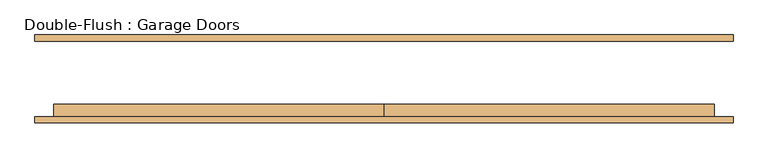
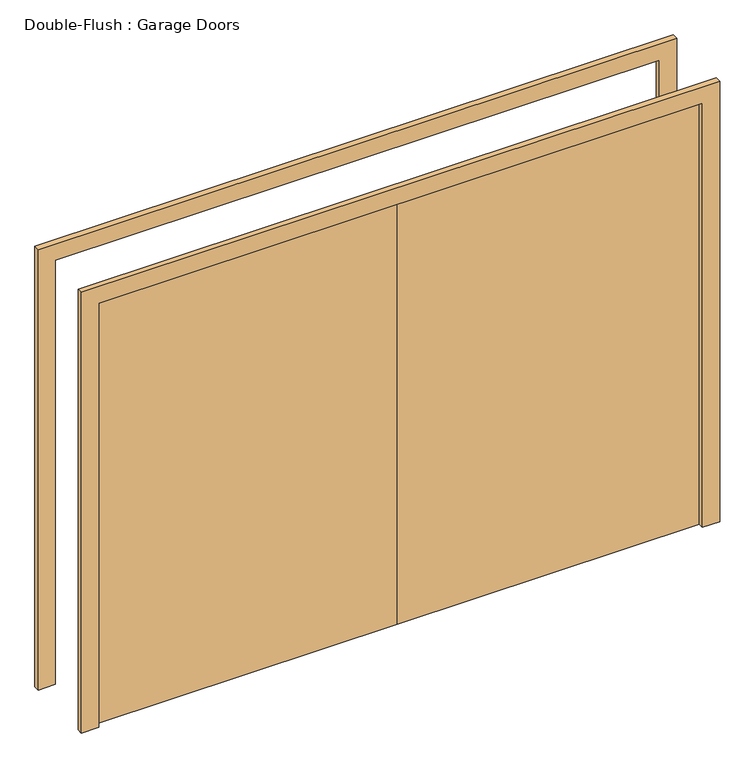
"""IFC4 building model written with IfcOpenShell, lengths in millimetres: door geometry, Double-Flush : Garage Doors."""

from ifc_helpers import new_model, si_unit, frame, origin, origin_with_axes, place, context, project, spatial, polyline, outline, extrude, source, transform, mapped, element, save


def double_flush_garage_doors_196828e7(model_context):
    return source(origin(), model_context, "Body", "SweptSolid", [
        extrude(outline(polyline([(0.0, -152.4), (0.0, -101.6), (1333.5, -101.6), (1333.5, -152.4), (0.0, -152.4)])), origin_with_axes(), (0.0, 0.0, 1.0), 1981.2),
        extrude(outline(polyline([(-1333.5, -152.4), (-1333.5, -101.6), (0.0, -101.6), (0.0, -152.4), (-1333.5, -152.4)])), origin_with_axes(), (0.0, 0.0, 1.0), 1981.2),
        extrude(outline(polyline([(1981.2, -1333.5), (1981.2, 1333.5), (0.0, 1333.5), (0.0, 1409.7), (2057.4, 1409.7), (2057.4, -1409.7), (0.0, -1409.7), (0.0, -1333.5), (1981.2, -1333.5)])), frame((0.0, 152.4, 0.0), z_axis=(0.0, 1.0, 0.0), x_axis=(0.0, 0.0, 1.0)), (0.0, 0.0, 1.0), 25.4),
        extrude(outline(polyline([(1981.2, -1333.5), (1981.2, 1333.5), (0.0, 1333.5), (0.0, 1409.7), (2057.4, 1409.7), (2057.4, -1409.7), (0.0, -1409.7), (0.0, -1333.5), (1981.2, -1333.5)])), frame((0.0, -177.8, 0.0), z_axis=(0.0, 1.0, 0.0), x_axis=(0.0, 0.0, 1.0)), (0.0, 0.0, 1.0), 25.4),
    ])


if __name__ == "__main__":
    model = new_model("IFC4")
    model_context = context("Model", 3, world=origin())
    ifc_project = project(units=[si_unit("LENGTHUNIT", "METRE", prefix="MILLI")], contexts=[model_context])
    site = spatial("IfcSite", under=ifc_project)
    building = spatial("IfcBuilding", under=site)
    placement = place(None, origin())
    double_flush_garage_doors_shape = double_flush_garage_doors_196828e7(model_context)
    element("IfcDoor", 1, ObjectType="Double-Flush : Garage Doors", at=placement, inside=building, context=model_context, shape_type="MappedRepresentation", body=[
        mapped(double_flush_garage_doors_shape, transform((0.0, 0.0, 0.0), x_axis=(1.0, 0.0, 0.0), y_axis=(0.0, 1.0, 0.0), z_axis=(0.0, 0.0, 1.0))),
    ])
    save(model, "model.ifc")

# Revit data of these elements
# Type "Double-Flush : Garage Doors"
#   Type Mark = "28"
#   Assembly Code = "C1020"
#   Thickness = 0' - 2"
#   Height = 6' - 6"
#   Trim Projection Ext = 0' - 1"
#   Trim Projection Int = 0' - 1"
#   Trim Width = 0' - 3"
#   Width = 8' - 9"
#   Function = 0
#   Door Material = Door - Panel
#   Frame Material = Concrete - Cast-in-Place Concrete
#   Wall Closure = (empty or 0)
# Element 1 (IfcDoor, "Double-Flush : Garage Doors")
#   Materials on its faces: "Concrete - Cast-in-Place Concrete", "Door - Panel"
# Materials
#   "Door - Panel": class "Wood", colour RGB 149 143 132, transparency 0, Comments = "Rendering appearance not upgraded Rendering appearance not upgraded "
#   "Concrete - Cast-in-Place Concrete": class "Concrete", colour RGB 178 178 178, transparency 0, Comments = "Rendering appearance not upgraded Rendering appearance not upgraded ", Description = "Concrete"
